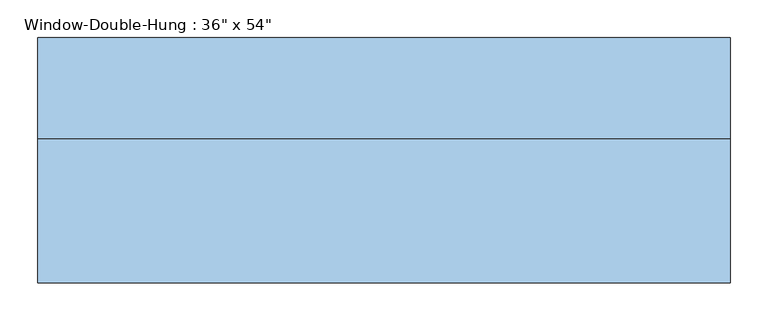
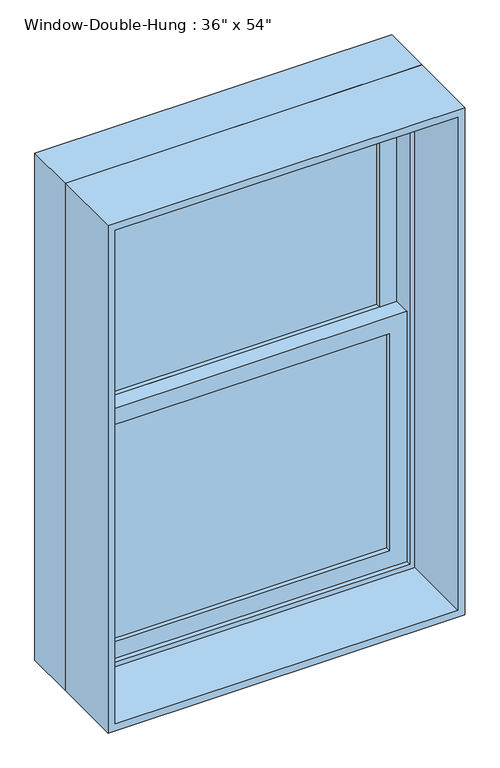
"""IFC4 building model written with IfcOpenShell, lengths in millimetres: window geometry."""

from ifc_helpers import new_model, si_unit, frame, origin, place, context, project, spatial, polyline, outline, extrude, source, transform, mapped, element, save


def window_0fbf8631(model_context):
    return source(origin(), model_context, "Body", "SweptSolid", [
        extrude(outline(polyline([(381.0, 82.55), (381.0, 76.2), (-381.0, 76.2), (-381.0, 82.55), (381.0, 82.55)])), frame((0.0, 0.0, 990.6), z_axis=(0.0, 0.0, 1.0), x_axis=(1.0, 0.0, 0.0)), (0.0, 0.0, 1.0), 587.375),
        extrude(outline(polyline([(-381.0, 69.85), (381.0, 69.85), (381.0, 63.5), (-381.0, 63.5), (-381.0, 69.85)])), frame((0.0, 0.0, 990.6), z_axis=(0.0, 0.0, 1.0), x_axis=(1.0, 0.0, 0.0)), (0.0, 0.0, 1.0), 587.375),
        extrude(outline(polyline([(381.0, 127.0), (381.0, 120.65), (-381.0, 120.65), (-381.0, 127.0), (381.0, 127.0)])), frame((0.0, 0.0, 1622.425), z_axis=(0.0, 0.0, 1.0), x_axis=(1.0, 0.0, 0.0)), (0.0, 0.0, 1.0), 587.375),
        extrude(outline(polyline([(-381.0, 114.3), (381.0, 114.3), (381.0, 107.95), (-381.0, 107.95), (-381.0, 114.3)])), frame((0.0, 0.0, 1622.425), z_axis=(0.0, 0.0, 1.0), x_axis=(1.0, 0.0, 0.0)), (0.0, 0.0, 1.0), 587.375),
        extrude(outline(polyline([(1622.425, -425.45), (946.15, -425.45), (946.15, 425.45), (1622.425, 425.45), (1622.425, -425.45)]), holes=[polyline([(1577.975, 381.0), (990.6, 381.0), (990.6, -381.0), (1577.975, -381.0), (1577.975, 381.0)])]), frame((0.0, 50.8, 0.0), z_axis=(0.0, 1.0, 0.0), x_axis=(0.0, 0.0, 1.0)), (0.0, 0.0, 1.0), 44.45),
        extrude(outline(polyline([(2254.25, -425.45), (1577.975, -425.45), (1577.975, 425.45), (2254.25, 425.45), (2254.25, -425.45)]), holes=[polyline([(2209.8, 381.0), (1622.425, 381.0), (1622.425, -381.0), (2209.8, -381.0), (2209.8, 381.0)])]), frame((0.0, 95.25, 0.0), z_axis=(0.0, 1.0, 0.0), x_axis=(0.0, 0.0, 1.0)), (0.0, 0.0, 1.0), 44.45),
        extrude(outline(polyline([(2286.0, -457.2), (914.4, -457.2), (914.4, 457.2), (2286.0, 457.2), (2286.0, -457.2)]), holes=[polyline([(2254.25, 425.45), (946.15, 425.45), (946.15, -425.45), (2254.25, -425.45), (2254.25, 425.45)])]), frame((0.0, 38.1, 0.0), z_axis=(0.0, 1.0, 0.0), x_axis=(0.0, 0.0, 1.0)), (0.0, 0.0, 1.0), 133.35),
        extrude(outline(polyline([(2286.0, 457.2), (2286.0, -457.2), (914.4, -457.2), (914.4, 457.2), (2286.0, 457.2)]), holes=[polyline([(2266.95, 438.15), (933.45, 438.15), (933.45, -438.15), (2266.95, -438.15), (2266.95, 438.15)])]), frame((0.0, -152.4, 0.0), z_axis=(0.0, 1.0, 0.0), x_axis=(0.0, 0.0, 1.0)), (0.0, 0.0, 1.0), 190.5),
    ])


if __name__ == "__main__":
    model = new_model("IFC4")
    model_context = context("Model", 3, world=origin())
    ifc_project = project(units=[si_unit("LENGTHUNIT", "METRE", prefix="MILLI")], contexts=[model_context])
    site = spatial("IfcSite", under=ifc_project)
    building = spatial("IfcBuilding", under=site)
    placement = place(None, origin())
    window_shape = window_0fbf8631(model_context)
    element("IfcWindow", 1, ObjectType="Window-Double-Hung : 36\" x 54\"", at=placement, inside=building, context=model_context, shape_type="MappedRepresentation", body=[
        mapped(window_shape, transform((0.0, 0.0, 0.0), x_axis=(1.0, 0.0, 0.0), y_axis=(0.0, 1.0, 0.0), z_axis=(0.0, 0.0, 1.0))),
    ])
    save(model, "model.ifc")

# Revit data of these elements
# Type "Window-Double-Hung : 36\" x 54\""
#   Type Mark = "18"
#   Fire Rating = "0.5h"
#   Construction Type Id = "DG-DR"
#   Assembly Code = "B2020100"
#   Analytic Construction = "Double glazing - domestic"
#   Wall Thickness [instance default] = 0' - 6"
#   Window Inset [instance default] = 0' - 0"
#   Visual Light Transmittance = 0.81
#   Thermal Resistance (R) = 1.8146 (h·ft²·°F)/BTU
#   Solar Heat Gain Coefficient = 0.76
#   Muntin Width = 2' - 6"
#   Muntin Height = 1' - 11 1/8"
#   Interior Wall Closure [instance default] = 0' - 1 1/2"
#   Rough Width = 3' - 0 1/2"
#   Rough Height = 4' - 6 1/2"
#   Frame Extension [instance default] = 0' - 1 1/4"
#   Exterior Wall Closure [instance default] = 0' - 0 1/2"
#   Extension Jamb [instance default] = 0' - 1 1/2"
#   Heat Transfer Coefficient (U) = 0.5511 BTU/(h·ft²·°F)
#   Height = 4' - 6"
#   Width = 3' - 0"
#   Top Muntin Visibility = yes
#   Indicator Visibility [instance default] = yes
#   Extension Jamb Visibility [instance default] = yes
#   Interior Trim Visibility [instance default] = yes
#   Exterior Trim Visibility [instance default] = yes
#   Define Thermal Properties by = 1
#   Bottom Muntin Visibility = yes
#   Muntin Pattern = Muntin Pattern_2x2 : Muntin Pattern_2x2
#   Interior Trim Material = Maple - Semigloss(Rotated)
#   Interior Trim = Trim-Window-Interior-Flat : Picture Frame
#   Exterior Trim Material = Clad - White
#   Exterior Trim = Trim-Window-Exterior-Flat : with Sill
#   Glass Panel Material = Glass, Clear Glazing
#   Exterior Frame Material = Clad - White
#   Interior Frame Material = Maple - Semigloss(Rotated)
#   Wall Closure = (empty or 0)
# Element 1 (IfcWindow, "Window-Double-Hung : 36\" x 54\"")
#   Wall Thickness = 1' - 0"
#   Extension Jamb = 0' - 7 1/2"
#   Materials on its faces: "Maple - Semigloss(Rotated)", "Glass, Clear Glazing", "Clad - White"
# Materials
#   "Maple - Semigloss(Rotated)": class "Wood", colour RGB 196 161 118, transparency 0, Description = "Acer Saccharum", Cost = 0
#   "Clad - White": class "Wood", colour RGB 245 245 243, transparency 0, Cost = 0
#   "Glass, Clear Glazing": class "Glass", colour RGB 245 245 243, transparency 1, Description = "Clear glazing", Cost = 0
